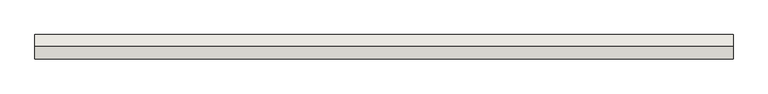
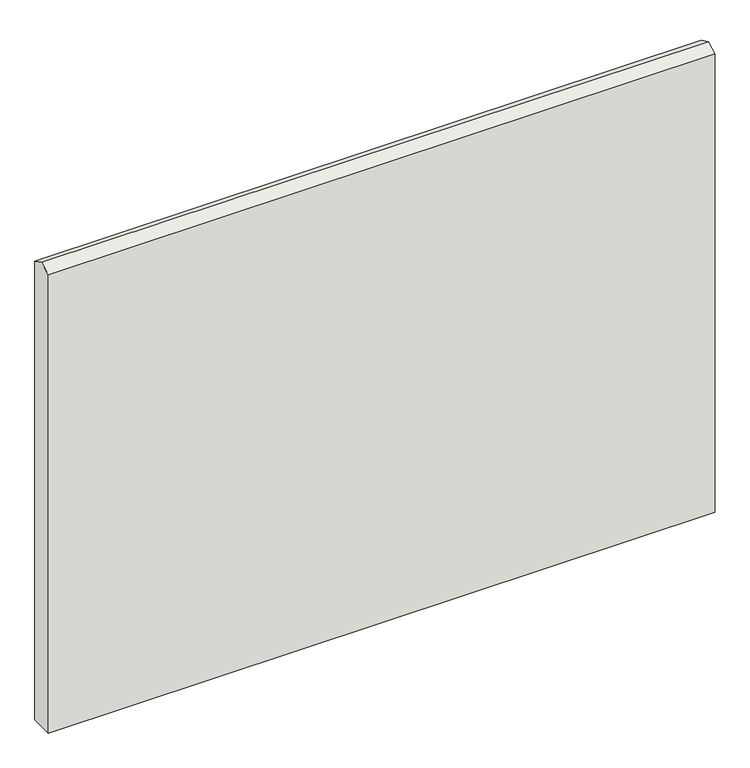
"""IFC4 building model written with IfcOpenShell, lengths in millimetres: wall geometry, Holzwand."""

from ifc_helpers import new_model, si_unit, frame, origin, place, context, project, spatial, polyline, outline, extrude, source, transform, mapped, element, save


def wall_7c4cc470(model_context):
    return source(origin(), model_context, "Body", "SweptSolid", [
        extrude(outline(polyline([(100.0, 4251.6781465), (200.0, 4200.7256015), (200.0, 0.0), (0.0, 0.0), (0.0, 4200.7256015), (100.0, 4251.6781465)])), frame((0.0, 0.0, 0.0), z_axis=(1.0, 0.0, 0.0), x_axis=(0.0, 1.0, 0.0)), (0.0, 0.0, 1.0), 5780.0),
    ])


if __name__ == "__main__":
    model = new_model("IFC4")
    model_context = context("Model", 3, world=origin())
    ifc_project = project(units=[si_unit("LENGTHUNIT", "METRE", prefix="MILLI")], contexts=[model_context])
    site = spatial("IfcSite", under=ifc_project)
    building = spatial("IfcBuilding", under=site)
    placement = place(None, origin())
    wall_shape = wall_7c4cc470(model_context)
    element("IfcWall", 1, ObjectType="Holzwand", at=placement, inside=building, context=model_context, shape_type="MappedRepresentation", body=[
        mapped(wall_shape, transform((0.0, 0.0, 0.0), x_axis=(1.0, 0.0, 0.0), y_axis=(0.0, 1.0, 0.0), z_axis=(0.0, 0.0, 1.0))),
    ])
    save(model, "model.ifc")

# Revit data of these elements
# Element 1 (IfcWall, "Holzwand")
#   Materials on its faces: "holzschalung"
# Materials
#   "holzschalung": class "Unassigned", colour RGB 128 128 128, transparency 0
